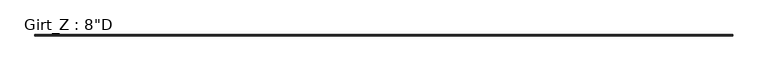
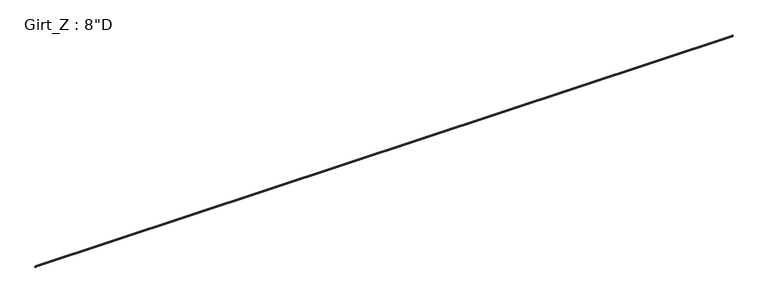
"""IFC4 building model written with IfcOpenShell, lengths in millimetres: beam geometry."""

import ifcopenshell
import ifcopenshell.guid

model = None  # the IFC model being written
_history = None  # IfcOwnerHistory: only IFC2X3 demands one
_inside = {}  # id of a spatial element -> (the spatial element, [elements in it])
_under = {}  # id of a project, library or spatial element -> (it, [spatial elements below it])
_declared = {}  # id of a project -> (the project, [libraries it declares])
_typed = {}  # id of a type object -> (the type object, [elements of that type])
_made_of = {}  # id of a material, layer set ... -> (it, [elements and type objects made of it])


def new_model(schema):
    """Start an empty IFC model of exactly this schema.

    Asked for "IFC4X3", IfcOpenShell would pick the latest addendum, in which some entities
    have other attributes; the version numbers below select the first issue.
    IFC2X3 requires an IfcOwnerHistory on every rooted entity: one is made here for all.
    """
    global model, _history
    if schema == "IFC4X3":
        model = ifcopenshell.file(schema_version=(4, 3, 0, 0))
    else:
        model = ifcopenshell.file(schema=schema)
    _inside.clear()
    _under.clear()
    _declared.clear()
    _typed.clear()
    _made_of.clear()
    _history = None
    if model.schema == "IFC2X3":
        org = make("IfcOrganization", Name="unknown")
        user = make(
            "IfcPersonAndOrganization",
            ThePerson=make("IfcPerson", FamilyName="unknown"),
            TheOrganization=org,
        )
        app = make(
            "IfcApplication",
            ApplicationDeveloper=org,
            Version="unknown",
            ApplicationFullName="unknown",
            ApplicationIdentifier="unknown",
        )
        _history = make(
            "IfcOwnerHistory",
            OwningUser=user,
            OwningApplication=app,
            ChangeAction="ADDED",
            CreationDate=0,
        )
    return model


def make(cls, **values):
    """One entity of the class cls with the attributes given. An attribute that is None is left unset."""
    return model.create_entity(
        cls, **{name: value for name, value in values.items() if value is not None}
    )


def rooted(cls, **values):
    """An entity with a GlobalId (a new one), such as an element, a storey or a relation."""
    return make(cls, GlobalId=ifcopenshell.guid.new(), OwnerHistory=_history, **values)


def si_unit(unit_type, name, prefix=None):
    """IfcSIUnit, for example si_unit("LENGTHUNIT", "METRE", prefix="MILLI")."""
    return make("IfcSIUnit", UnitType=unit_type, Prefix=prefix, Name=name)


def assignment(units):
    """IfcUnitAssignment: the units of a project."""
    return None if units is None else make("IfcUnitAssignment", Units=units)


def point(xyz):
    """IfcCartesianPoint."""
    return None if xyz is None else make("IfcCartesianPoint", Coordinates=xyz)


def direction(xyz):
    """IfcDirection."""
    return None if xyz is None else make("IfcDirection", DirectionRatios=xyz)


def frame(location, z_axis=None, x_axis=None):
    """IfcAxis2Placement3D, a coordinate frame: its origin and axes. An axis left out is left unset."""
    return make(
        "IfcAxis2Placement3D",
        Location=point(location),
        Axis=direction(z_axis),
        RefDirection=direction(x_axis),
    )


def frame_2d(location, x_axis=None):
    """IfcAxis2Placement2D, a coordinate frame in the plane: its origin and x axis."""
    return make(
        "IfcAxis2Placement2D", Location=point(location), RefDirection=direction(x_axis)
    )


def origin():
    """The frame at (0, 0, 0) with its axes left unset."""
    return frame((0.0, 0.0, 0.0))


def place(relative_to, where):
    """IfcLocalPlacement: puts the frame where relative to a parent placement (None: the world)."""
    return make(
        "IfcLocalPlacement", PlacementRelTo=relative_to, RelativePlacement=where
    )


def context(
    kind, dimensions, precision=None, world=None, true_north=None, identifier=None
):
    """IfcGeometricRepresentationContext, for example the 3D "Model" context."""
    return make(
        "IfcGeometricRepresentationContext",
        ContextIdentifier=identifier,
        ContextType=kind,
        CoordinateSpaceDimension=dimensions,
        Precision=precision,
        WorldCoordinateSystem=world,
        TrueNorth=true_north,
    )


def project(units=None, contexts=None):
    """IfcProject with its units and contexts."""
    return rooted(
        "IfcProject",
        Name="project",
        RepresentationContexts=contexts,
        UnitsInContext=assignment(units),
    )


def spatial(cls, under=None, at=None, **own):
    """A site, building, storey or space (cls), placed at a placement, below another one or the project."""
    s = rooted(cls, ObjectPlacement=at, **own)
    if under is not None:
        _under.setdefault(under.id(), (under, []))[1].append(s)
    return s


def polyline(points):
    """IfcPolyline through the points."""
    return make("IfcPolyline", Points=[point(p) for p in points])


def circle_curve(where, radius):
    """IfcCircle in the frame where."""
    return make("IfcCircle", Position=where, Radius=radius)


def trimmed(basis, trim1, trim2, sense, master):
    """IfcTrimmedCurve: the piece of a basis curve between two trims."""
    return make(
        "IfcTrimmedCurve",
        BasisCurve=basis,
        Trim1=trim1,
        Trim2=trim2,
        SenseAgreement=sense,
        MasterRepresentation=master,
    )


def segment(curve, same_sense, transition):
    """IfcCompositeCurveSegment."""
    return make(
        "IfcCompositeCurveSegment",
        Transition=transition,
        SameSense=same_sense,
        ParentCurve=curve,
    )


def composite_curve(segments, self_intersect=None):
    """IfcCompositeCurve: segments joined end to end."""
    return make("IfcCompositeCurve", Segments=segments, SelfIntersect=self_intersect)


def outline(outer, holes=None, kind="AREA"):
    """IfcArbitraryClosedProfileDef: a profile drawn as a closed curve; with holes, ...WithVoids."""
    if holes is None:
        return make("IfcArbitraryClosedProfileDef", ProfileType=kind, OuterCurve=outer)
    return make(
        "IfcArbitraryProfileDefWithVoids",
        ProfileType=kind,
        OuterCurve=outer,
        InnerCurves=holes,
    )


def extrude(swept, where, along, depth):
    """IfcExtrudedAreaSolid: the profile swept, set in the frame where, extruded along a direction by depth."""
    return make(
        "IfcExtrudedAreaSolid",
        SweptArea=swept,
        Position=where,
        ExtrudedDirection=direction(along),
        Depth=depth,
    )


def shape(context_of_items, identifier, shape_type, items):
    """IfcShapeRepresentation: the items that make up one representation, for example the "Body"."""
    return make(
        "IfcShapeRepresentation",
        ContextOfItems=context_of_items,
        RepresentationIdentifier=identifier,
        RepresentationType=shape_type,
        Items=items,
    )


def source(mapping_origin, context_of_items, identifier, shape_type, items):
    """IfcRepresentationMap: a shape defined once, which mapped items show again and again."""
    return make(
        "IfcRepresentationMap",
        MappingOrigin=mapping_origin,
        MappedRepresentation=shape(context_of_items, identifier, shape_type, items),
    )


def transform(
    local_origin,
    x_axis=None,
    y_axis=None,
    z_axis=None,
    scale=None,
    scale2=None,
    scale3=None,
    uniform=True,
):
    """IfcCartesianTransformationOperator3D, or its non-uniform kind. x_axis, y_axis, z_axis: its Axis1, 2, 3."""
    if uniform:
        return make(
            "IfcCartesianTransformationOperator3D",
            Axis1=direction(x_axis),
            Axis2=direction(y_axis),
            LocalOrigin=point(local_origin),
            Scale=scale,
            Axis3=direction(z_axis),
        )
    return make(
        "IfcCartesianTransformationOperator3DnonUniform",
        Axis1=direction(x_axis),
        Axis2=direction(y_axis),
        LocalOrigin=point(local_origin),
        Scale=scale,
        Axis3=direction(z_axis),
        Scale2=scale2,
        Scale3=scale3,
    )


def mapped(mapping_source, mapping_target):
    """IfcMappedItem: shows the shape of a source again, moved by a transform."""
    return make(
        "IfcMappedItem", MappingSource=mapping_source, MappingTarget=mapping_target
    )


def made_of(thing, what):
    """Note that an element or type object is made of a material, layer set ...; save() writes the relation."""
    if what is not None:
        _made_of.setdefault(what.id(), (what, []))[1].append(thing)
    return thing


def element(
    cls,
    number,
    at=None,
    inside=None,
    cuts=None,
    type_object=None,
    material=None,
    context=None,
    identifier="Body",
    shape_type=None,
    held_by="IfcProductDefinitionShape",
    body=None,
    shapes=None,
    **own,
):
    """One element of the class cls, such as IfcWall. Its Tag is "e" and its number.

    at: its placement. inside: the storey or other place that contains it. cuts: it is an
    opening in that element (IfcRelVoidsElement). A single representation is given by context,
    identifier, shape_type and body (its items); several are given by shapes. held_by: the class
    of the entity that holds the representations. save() writes the other relations.
    """
    e = rooted(cls, Tag="e%d" % number, ObjectPlacement=at, **own)
    if body is not None:
        shapes = [shape(context, identifier, shape_type, body)]
    if shapes is not None:
        e.Representation = make(held_by, Representations=shapes)
    if inside is not None:
        _inside.setdefault(inside.id(), (inside, []))[1].append(e)
    if cuts is not None:
        rooted(
            "IfcRelVoidsElement", RelatingBuildingElement=cuts, RelatedOpeningElement=e
        )
    if type_object is not None:
        _typed.setdefault(type_object.id(), (type_object, []))[1].append(e)
    return made_of(e, material)


def aggregate(whole, parts):
    """IfcRelAggregates: a whole, such as a stair, and the parts it consists of."""
    return rooted("IfcRelAggregates", RelatingObject=whole, RelatedObjects=parts)


def save(model, path):
    """Write the relations noted so far, then the file.

    IfcRelAggregates (storeys below a building ...), IfcRelContainedInSpatialStructure (elements
    in a storey), IfcRelDefinesByType, IfcRelAssociatesMaterial and IfcRelDeclares: one each for
    every whole, place, type object, material and project.
    """
    for whole, parts in _under.values():
        aggregate(whole, parts)
    for where, things in _inside.values():
        rooted(
            "IfcRelContainedInSpatialStructure",
            RelatedElements=things,
            RelatingStructure=where,
        )
    for kind, things in _typed.values():
        rooted("IfcRelDefinesByType", RelatedObjects=things, RelatingType=kind)
    for what, things in _made_of.values():
        rooted("IfcRelAssociatesMaterial", RelatedObjects=things, RelatingMaterial=what)
    for by, libraries in _declared.values():
        rooted("IfcRelDeclares", RelatingContext=by, RelatedDefinitions=libraries)
    model.write(path)


def beam_b138bea9(model_context):
    return source(origin(), model_context, "Body", "SweptSolid", [
        extrude(outline(composite_curve([segment(polyline([(-63.5, 101.6), (-3.3734375, 101.6)]), True, "CONTINUOUS"), segment(trimmed(circle_curve(frame_2d((-3.3734375, 96.8375)), 4.7625), [point((-3.3734375, 101.6))], [point((1.3890625, 96.8375))], False, "CARTESIAN"), True, "CONTINUOUS"), segment(polyline([(1.3890625, 96.8375), (1.3890625, -96.8389339)]), True, "CONTINUOUS"), segment(trimmed(circle_curve(frame_2d((3.3748024, -96.8389339)), 1.9857399), [point((1.3890625, -96.8389339))], [point((3.2694106, -98.821875))], True, "CARTESIAN"), True, "CONTINUOUS"), segment(polyline([(3.2694106, -98.821875), (62.204539, -98.821875), (73.6169367, -85.221109), (75.745104, -87.0068534), (63.5, -101.6), (3.3734375, -101.6)]), True, "CONTINUOUS"), segment(trimmed(circle_curve(frame_2d((3.3734375, -96.8375)), 4.7625), [point((3.3734375, -101.6))], [point((-1.3890625, -96.8375))], False, "CARTESIAN"), True, "CONTINUOUS"), segment(polyline([(-1.3890625, -96.8375), (-1.3890625, 96.8381931)]), True, "CONTINUOUS"), segment(trimmed(circle_curve(frame_2d((-3.3741066, 96.8381931)), 1.9850441), [point((-1.3890625, 96.8381931))], [point((-3.3005807, 98.821875))], True, "CARTESIAN"), True, "CONTINUOUS"), segment(polyline([(-3.3005807, 98.821875), (-62.204539, 98.821875), (-73.6169367, 85.221109), (-75.745104, 87.0068534), (-63.5, 101.6)]), True, "CONTINUOUS")], self_intersect=False)), frame((-40574.7884766, 0.0, 0.0), z_axis=(1.0, 0.0, 0.0), x_axis=(0.0, 1.0, 0.0)), (0.0, 0.0, 1.0), 80730.4769531),
    ])


if __name__ == "__main__":
    model = new_model("IFC4")
    model_context = context("Model", 3, world=origin())
    ifc_project = project(units=[si_unit("LENGTHUNIT", "METRE", prefix="MILLI")], contexts=[model_context])
    site = spatial("IfcSite", under=ifc_project)
    building = spatial("IfcBuilding", under=site)
    placement = place(None, origin())
    beam_shape = beam_b138bea9(model_context)
    element("IfcBeam", 1, ObjectType="Girt_Z : 8\"D", at=placement, inside=building, context=model_context, shape_type="MappedRepresentation", body=[
        mapped(beam_shape, transform((0.0, 0.0, 0.0), x_axis=(1.0, 0.0, 0.0), y_axis=(0.0, 1.0, 0.0), z_axis=(0.0, 0.0, 1.0))),
    ])
    save(model, "model.ifc")

# Revit data of these elements
# Type "Girt_Z : 8\"D"
#   Web_Thickness = 0' - 0 7/64"
#   Length [instance default] = 10' - 0"
#   Leg_1 = 0' - 2 1/2"
#   Height = 0' - 8"
#   Structural Material [instance default] = none
# Element 1 (IfcBeam, "Girt_Z : 8\"D")
#   Structural Material = Steel
#   Materials on its faces: "Steel"
# Materials
#   "Steel": class "Metal", colour RGB 118 118 114, transparency 0, Description = "Steel, mill finish", Cost = 0
